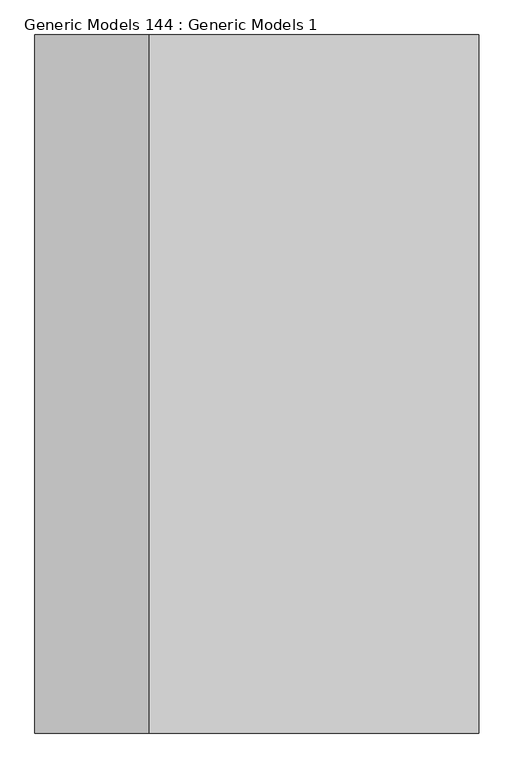
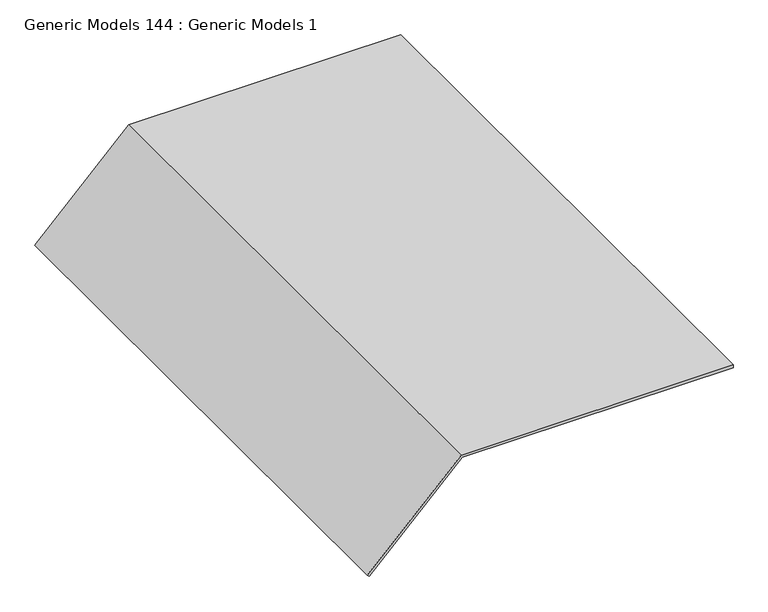
"""IFC4 building model written with IfcOpenShell, lengths in millimetres: proxy geometry, Generic Models 144 : Generic Models 1."""

from ifc_helpers import new_model, si_unit, frame, origin, place, context, project, spatial, polyline, outline, extrude, source, transform, mapped, element, save


def generic_models_144_generic_models_1_4ebe4832(model_context):
    return source(origin(), model_context, "Body", "SweptSolid", [
        extrude(outline(polyline([(-79.375, 52785.9625), (-73.025, 52785.9625), (-73.025, 52209.6280698), (-272.1843039, 52010.4687659), (-276.674432, 52014.9588939), (-79.375, 52212.2583259), (-79.375, 52785.9625)])), frame((0.0, 0.0, 0.0), z_axis=(0.0, 1.0, 0.0), x_axis=(0.0, 0.0, 1.0)), (0.0, 0.0, 1.0), 1219.2),
    ])


if __name__ == "__main__":
    model = new_model("IFC4")
    model_context = context("Model", 3, world=origin())
    ifc_project = project(units=[si_unit("LENGTHUNIT", "METRE", prefix="MILLI")], contexts=[model_context])
    site = spatial("IfcSite", under=ifc_project)
    building = spatial("IfcBuilding", under=site)
    placement = place(None, origin())
    generic_models_144_generic_models_1_shape = generic_models_144_generic_models_1_4ebe4832(model_context)
    element("IfcBuildingElementProxy", 1, Name="Generic Models 144 : Generic Models 1", ObjectType="Generic Models 144 : Generic Models 1", at=placement, inside=building, context=model_context, shape_type="MappedRepresentation", body=[
        mapped(generic_models_144_generic_models_1_shape, transform((0.0, 0.0, 0.0), x_axis=(1.0, 0.0, 0.0), y_axis=(0.0, 1.0, 0.0), z_axis=(0.0, 0.0, 1.0))),
    ])
    save(model, "model.ifc")

# Revit data of these elements
# Element 1 (IfcBuildingElementProxy, "Generic Models 144 : Generic Models 1")
#   Materials on its faces: "#10 6x6 WIRE MESH"
# Materials
#   "#10 6x6 WIRE MESH": class "Metal", colour RGB 189 187 185, transparency 0, Description = "Structural steel 50ksi", Cost = 0
